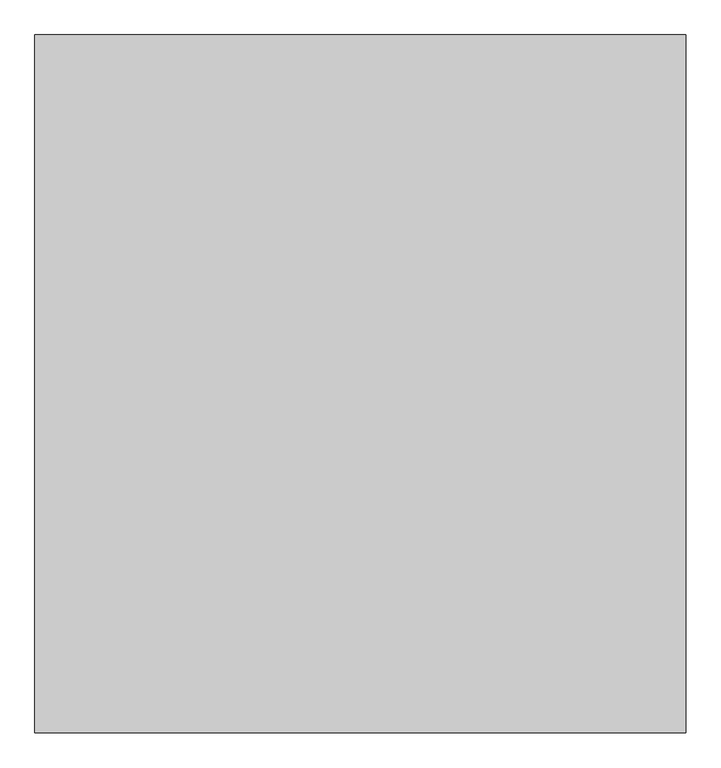
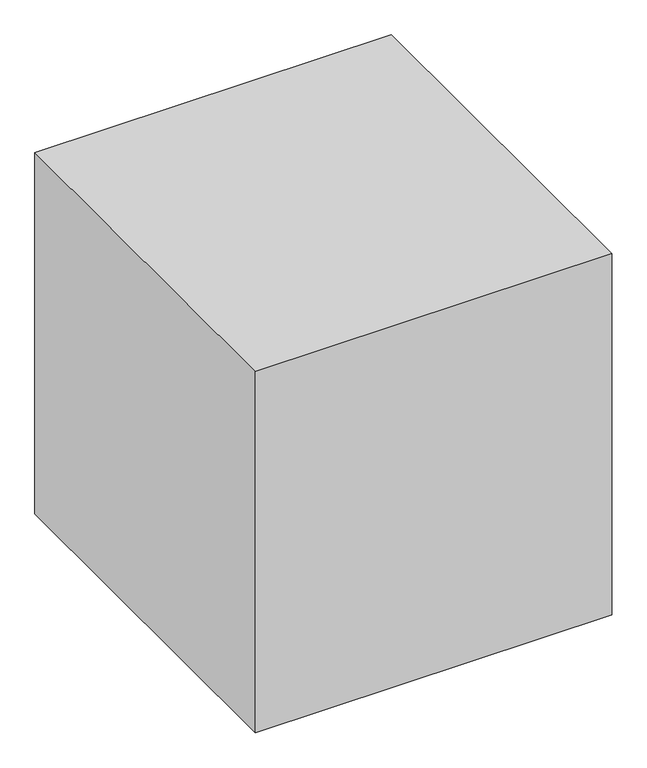
"""IFC4 building model written with IfcOpenShell, lengths in millimetres: proxy geometry, Space Planning Box_hec : Space Planning Box_hec."""

from ifc_helpers import new_model, si_unit, origin, origin_with_axes, place, context, project, spatial, polyline, outline, extrude, source, transform, mapped, element, save


def generic_models_ec17d728(model_context):
    return source(origin(), model_context, "Body", "SweptSolid", [
        extrude(outline(polyline([(2800.0, 3000.0), (2800.0, -3000.0), (-2800.0, -3000.0), (-2800.0, 3000.0), (2800.0, 3000.0)])), origin_with_axes(), (0.0, 0.0, 1.0), 6000.0),
    ])


if __name__ == "__main__":
    model = new_model("IFC4")
    model_context = context("Model", 3, world=origin())
    ifc_project = project(units=[si_unit("LENGTHUNIT", "METRE", prefix="MILLI")], contexts=[model_context])
    site = spatial("IfcSite", under=ifc_project)
    building = spatial("IfcBuilding", under=site)
    placement = place(None, origin())
    generic_models_shape = generic_models_ec17d728(model_context)
    element("IfcBuildingElementProxy", 1, Name="Space Planning Box_hec : Space Planning Box_hec", ObjectType="Space Planning Box_hec : Space Planning Box_hec", at=placement, inside=building, context=model_context, shape_type="MappedRepresentation", body=[
        mapped(generic_models_shape, transform((0.0, 0.0, 0.0), x_axis=(1.0, 0.0, 0.0), y_axis=(0.0, 1.0, 0.0), z_axis=(0.0, 0.0, 1.0))),
    ])
    save(model, "model.ifc")

# Revit data of these elements
# Type "Space Planning Box_hec : Space Planning Box_hec"
#   Type Comments = "..."
#   Room Name [instance default] = "?"
#   Interior Finish [instance default] = ""
#   Exterior Finish [instance default] = ""
#   Department [instance default] = ""
#   Assembly Code = "..."
#   Width [instance default] = 1524 mm
#   Program Area [instance default] = 0 m²
#   Length [instance default] = 1524 mm
#   Height [instance default] = 1524 mm
#   Area [instance default] = 2.32258 m²
#   Fill Color [instance default] = Cyan
#   Default Elevation = 0
# Element 1 (IfcBuildingElementProxy, "Space Planning Box_hec : Space Planning Box_hec")
#   Room Name = "Locker Room (M)"
#   Interior Finish = "IF2-1"
#   Exterior Finish = "EF1"
#   Department = "AR"
#   Width = 5600 mm
#   Program Area = 31.5 m²
#   Length = 6000 mm
#   Height = 6000 mm
#   Area = 33.6 m²
#   Fill Color = Lavender
#   Materials on its faces: "Lavender"
# Materials
#   "Cyan": class "Generic", colour RGB 0 255 255, transparency 0.2, Cost = 0
#   "Lavender": class "Generic", colour RGB 186 85 211, transparency 0.2, Cost = 0
